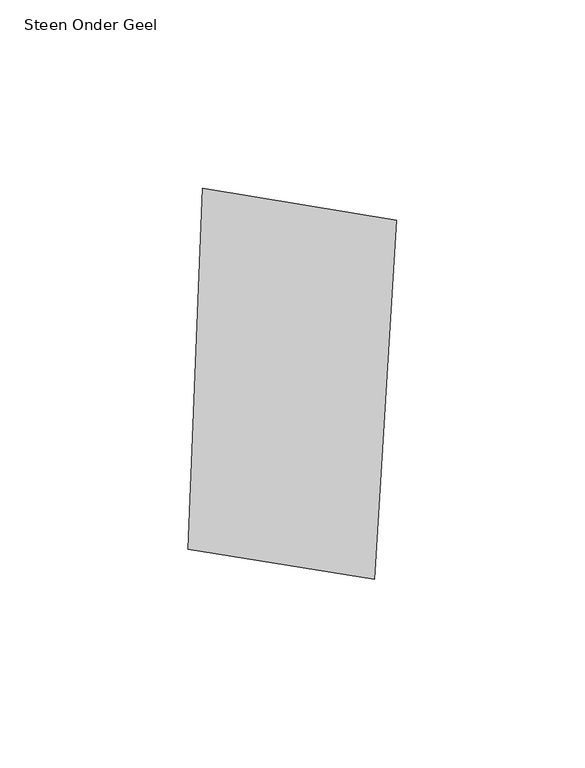
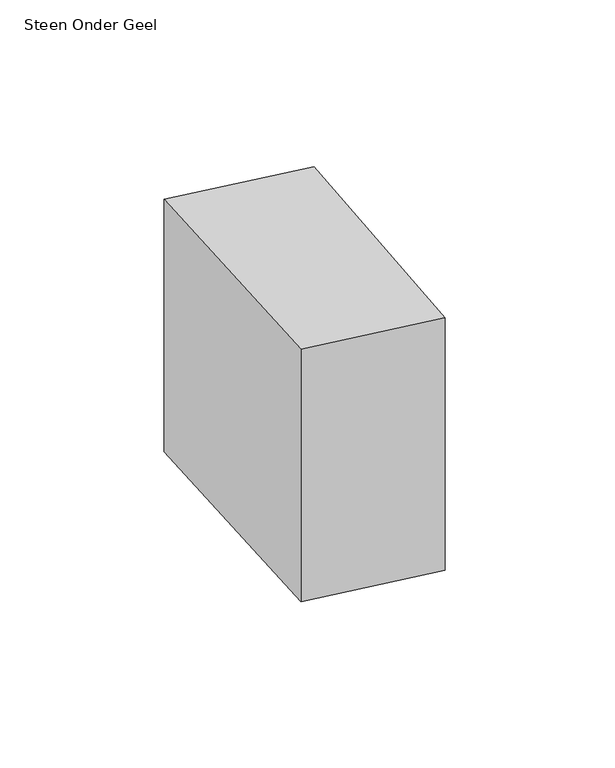
"""IFC4 building model written with IfcOpenShell, lengths in millimetres: proxy geometry, 00_GMA_steen_versie_4 : Steen Onder Geel."""

from ifc_helpers import new_model, si_unit, origin, origin_with_axes, place, context, project, spatial, polyline, outline, extrude, source, transform, mapped, element, save


def steen_onder_geel_8fa2c960(model_context):
    return source(origin(), model_context, "Body", "SweptSolid", [
        extrude(outline(polyline([(103.415686, 114.5642242), (97.5118052, 19.2471637), (48.1626706, 27.2884889), (51.9825501, 122.9554339), (103.415686, 114.5642242)])), origin_with_axes(), (0.0, 0.0, 1.0), 100.0),
    ])


if __name__ == "__main__":
    model = new_model("IFC4")
    model_context = context("Model", 3, world=origin())
    ifc_project = project(units=[si_unit("LENGTHUNIT", "METRE", prefix="MILLI")], contexts=[model_context])
    site = spatial("IfcSite", under=ifc_project)
    building = spatial("IfcBuilding", under=site)
    placement = place(None, origin())
    steen_onder_geel_shape = steen_onder_geel_8fa2c960(model_context)
    element("IfcBuildingElementProxy", 1, Name="00_GMA_steen_versie_4 : Steen Onder Geel", ObjectType="00_GMA_steen_versie_4 : Steen Onder Geel", at=placement, inside=building, context=model_context, shape_type="MappedRepresentation", body=[
        mapped(steen_onder_geel_shape, transform((0.0, 0.0, 0.0), x_axis=(1.0, 0.0, 0.0), y_axis=(0.0, 1.0, 0.0), z_axis=(0.0, 0.0, 1.0))),
    ])
    save(model, "model.ifc")

# Revit data of these elements
# Type "00_GMA_steen_versie_4 : Steen Onder Geel"
#   StootVoegHalfBoven [instance default] = 5 mm
#   StootVoegHalf [instance default] = 5 mm
#   StootVoegBreedteOnder = 10 mm
#   StootVoegBreedteBoven = 10 mm
#   Steendikte = 100 mm
#   LintVoegOnderHalf = 0 mm
#   LintVoegOnder = 0 mm
#   LintVoegBovenHalf = 5 mm
#   LintVoegBoven = 10 mm
#   materiaal = 21_steen_geel
#   MateriaalVoeg = none
#   Default Elevation = 0
# Element 1 (IfcBuildingElementProxy, "00_GMA_steen_versie_4 : Steen Onder Geel")
#   Materials on its faces: "21_steen_geel"
# Materials
#   "21_steen_geel": class "Unassigned", colour RGB 202 202 0, transparency 0, Cost = 0
